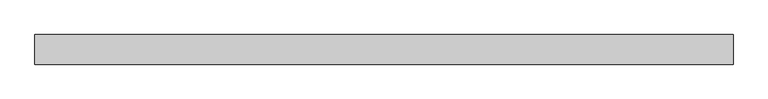
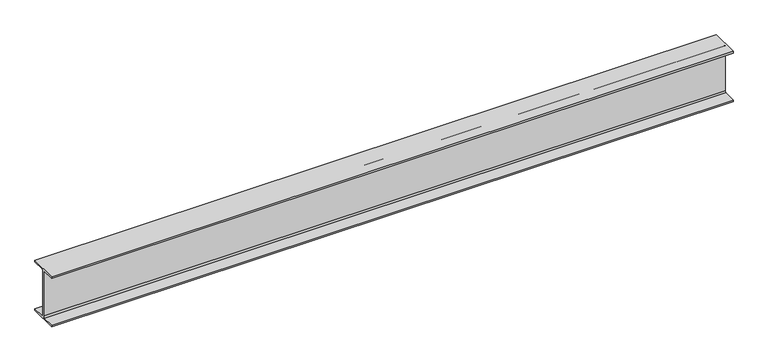
"""IFC4 building model written with IfcOpenShell, lengths in millimetres: beam geometry, Old_Steel Beam_H-KSD3502 : H_SB_ASB_H-250×125x6x9."""

import ifcopenshell
import ifcopenshell.guid

model = None  # the IFC model being written
_history = None  # IfcOwnerHistory: only IFC2X3 demands one
_inside = {}  # id of a spatial element -> (the spatial element, [elements in it])
_under = {}  # id of a project, library or spatial element -> (it, [spatial elements below it])
_declared = {}  # id of a project -> (the project, [libraries it declares])
_typed = {}  # id of a type object -> (the type object, [elements of that type])
_made_of = {}  # id of a material, layer set ... -> (it, [elements and type objects made of it])


def new_model(schema):
    """Start an empty IFC model of exactly this schema.

    Asked for "IFC4X3", IfcOpenShell would pick the latest addendum, in which some entities
    have other attributes; the version numbers below select the first issue.
    IFC2X3 requires an IfcOwnerHistory on every rooted entity: one is made here for all.
    """
    global model, _history
    if schema == "IFC4X3":
        model = ifcopenshell.file(schema_version=(4, 3, 0, 0))
    else:
        model = ifcopenshell.file(schema=schema)
    _inside.clear()
    _under.clear()
    _declared.clear()
    _typed.clear()
    _made_of.clear()
    _history = None
    if model.schema == "IFC2X3":
        org = make("IfcOrganization", Name="unknown")
        user = make(
            "IfcPersonAndOrganization",
            ThePerson=make("IfcPerson", FamilyName="unknown"),
            TheOrganization=org,
        )
        app = make(
            "IfcApplication",
            ApplicationDeveloper=org,
            Version="unknown",
            ApplicationFullName="unknown",
            ApplicationIdentifier="unknown",
        )
        _history = make(
            "IfcOwnerHistory",
            OwningUser=user,
            OwningApplication=app,
            ChangeAction="ADDED",
            CreationDate=0,
        )
    return model


def make(cls, **values):
    """One entity of the class cls with the attributes given. An attribute that is None is left unset."""
    return model.create_entity(
        cls, **{name: value for name, value in values.items() if value is not None}
    )


def rooted(cls, **values):
    """An entity with a GlobalId (a new one), such as an element, a storey or a relation."""
    return make(cls, GlobalId=ifcopenshell.guid.new(), OwnerHistory=_history, **values)


def si_unit(unit_type, name, prefix=None):
    """IfcSIUnit, for example si_unit("LENGTHUNIT", "METRE", prefix="MILLI")."""
    return make("IfcSIUnit", UnitType=unit_type, Prefix=prefix, Name=name)


def assignment(units):
    """IfcUnitAssignment: the units of a project."""
    return None if units is None else make("IfcUnitAssignment", Units=units)


def point(xyz):
    """IfcCartesianPoint."""
    return None if xyz is None else make("IfcCartesianPoint", Coordinates=xyz)


def direction(xyz):
    """IfcDirection."""
    return None if xyz is None else make("IfcDirection", DirectionRatios=xyz)


def frame(location, z_axis=None, x_axis=None):
    """IfcAxis2Placement3D, a coordinate frame: its origin and axes. An axis left out is left unset."""
    return make(
        "IfcAxis2Placement3D",
        Location=point(location),
        Axis=direction(z_axis),
        RefDirection=direction(x_axis),
    )


def frame_2d(location, x_axis=None):
    """IfcAxis2Placement2D, a coordinate frame in the plane: its origin and x axis."""
    return make(
        "IfcAxis2Placement2D", Location=point(location), RefDirection=direction(x_axis)
    )


def origin():
    """The frame at (0, 0, 0) with its axes left unset."""
    return frame((0.0, 0.0, 0.0))


def place(relative_to, where):
    """IfcLocalPlacement: puts the frame where relative to a parent placement (None: the world)."""
    return make(
        "IfcLocalPlacement", PlacementRelTo=relative_to, RelativePlacement=where
    )


def context(
    kind, dimensions, precision=None, world=None, true_north=None, identifier=None
):
    """IfcGeometricRepresentationContext, for example the 3D "Model" context."""
    return make(
        "IfcGeometricRepresentationContext",
        ContextIdentifier=identifier,
        ContextType=kind,
        CoordinateSpaceDimension=dimensions,
        Precision=precision,
        WorldCoordinateSystem=world,
        TrueNorth=true_north,
    )


def project(units=None, contexts=None):
    """IfcProject with its units and contexts."""
    return rooted(
        "IfcProject",
        Name="project",
        RepresentationContexts=contexts,
        UnitsInContext=assignment(units),
    )


def spatial(cls, under=None, at=None, **own):
    """A site, building, storey or space (cls), placed at a placement, below another one or the project."""
    s = rooted(cls, ObjectPlacement=at, **own)
    if under is not None:
        _under.setdefault(under.id(), (under, []))[1].append(s)
    return s


def polyline(points):
    """IfcPolyline through the points."""
    return make("IfcPolyline", Points=[point(p) for p in points])


def circle_curve(where, radius):
    """IfcCircle in the frame where."""
    return make("IfcCircle", Position=where, Radius=radius)


def trimmed(basis, trim1, trim2, sense, master):
    """IfcTrimmedCurve: the piece of a basis curve between two trims."""
    return make(
        "IfcTrimmedCurve",
        BasisCurve=basis,
        Trim1=trim1,
        Trim2=trim2,
        SenseAgreement=sense,
        MasterRepresentation=master,
    )


def segment(curve, same_sense, transition):
    """IfcCompositeCurveSegment."""
    return make(
        "IfcCompositeCurveSegment",
        Transition=transition,
        SameSense=same_sense,
        ParentCurve=curve,
    )


def composite_curve(segments, self_intersect=None):
    """IfcCompositeCurve: segments joined end to end."""
    return make("IfcCompositeCurve", Segments=segments, SelfIntersect=self_intersect)


def outline(outer, holes=None, kind="AREA"):
    """IfcArbitraryClosedProfileDef: a profile drawn as a closed curve; with holes, ...WithVoids."""
    if holes is None:
        return make("IfcArbitraryClosedProfileDef", ProfileType=kind, OuterCurve=outer)
    return make(
        "IfcArbitraryProfileDefWithVoids",
        ProfileType=kind,
        OuterCurve=outer,
        InnerCurves=holes,
    )


def extrude(swept, where, along, depth):
    """IfcExtrudedAreaSolid: the profile swept, set in the frame where, extruded along a direction by depth."""
    return make(
        "IfcExtrudedAreaSolid",
        SweptArea=swept,
        Position=where,
        ExtrudedDirection=direction(along),
        Depth=depth,
    )


def shape(context_of_items, identifier, shape_type, items):
    """IfcShapeRepresentation: the items that make up one representation, for example the "Body"."""
    return make(
        "IfcShapeRepresentation",
        ContextOfItems=context_of_items,
        RepresentationIdentifier=identifier,
        RepresentationType=shape_type,
        Items=items,
    )


def source(mapping_origin, context_of_items, identifier, shape_type, items):
    """IfcRepresentationMap: a shape defined once, which mapped items show again and again."""
    return make(
        "IfcRepresentationMap",
        MappingOrigin=mapping_origin,
        MappedRepresentation=shape(context_of_items, identifier, shape_type, items),
    )


def transform(
    local_origin,
    x_axis=None,
    y_axis=None,
    z_axis=None,
    scale=None,
    scale2=None,
    scale3=None,
    uniform=True,
):
    """IfcCartesianTransformationOperator3D, or its non-uniform kind. x_axis, y_axis, z_axis: its Axis1, 2, 3."""
    if uniform:
        return make(
            "IfcCartesianTransformationOperator3D",
            Axis1=direction(x_axis),
            Axis2=direction(y_axis),
            LocalOrigin=point(local_origin),
            Scale=scale,
            Axis3=direction(z_axis),
        )
    return make(
        "IfcCartesianTransformationOperator3DnonUniform",
        Axis1=direction(x_axis),
        Axis2=direction(y_axis),
        LocalOrigin=point(local_origin),
        Scale=scale,
        Axis3=direction(z_axis),
        Scale2=scale2,
        Scale3=scale3,
    )


def mapped(mapping_source, mapping_target):
    """IfcMappedItem: shows the shape of a source again, moved by a transform."""
    return make(
        "IfcMappedItem", MappingSource=mapping_source, MappingTarget=mapping_target
    )


def made_of(thing, what):
    """Note that an element or type object is made of a material, layer set ...; save() writes the relation."""
    if what is not None:
        _made_of.setdefault(what.id(), (what, []))[1].append(thing)
    return thing


def element(
    cls,
    number,
    at=None,
    inside=None,
    cuts=None,
    type_object=None,
    material=None,
    context=None,
    identifier="Body",
    shape_type=None,
    held_by="IfcProductDefinitionShape",
    body=None,
    shapes=None,
    **own,
):
    """One element of the class cls, such as IfcWall. Its Tag is "e" and its number.

    at: its placement. inside: the storey or other place that contains it. cuts: it is an
    opening in that element (IfcRelVoidsElement). A single representation is given by context,
    identifier, shape_type and body (its items); several are given by shapes. held_by: the class
    of the entity that holds the representations. save() writes the other relations.
    """
    e = rooted(cls, Tag="e%d" % number, ObjectPlacement=at, **own)
    if body is not None:
        shapes = [shape(context, identifier, shape_type, body)]
    if shapes is not None:
        e.Representation = make(held_by, Representations=shapes)
    if inside is not None:
        _inside.setdefault(inside.id(), (inside, []))[1].append(e)
    if cuts is not None:
        rooted(
            "IfcRelVoidsElement", RelatingBuildingElement=cuts, RelatedOpeningElement=e
        )
    if type_object is not None:
        _typed.setdefault(type_object.id(), (type_object, []))[1].append(e)
    return made_of(e, material)


def aggregate(whole, parts):
    """IfcRelAggregates: a whole, such as a stair, and the parts it consists of."""
    return rooted("IfcRelAggregates", RelatingObject=whole, RelatedObjects=parts)


def save(model, path):
    """Write the relations noted so far, then the file.

    IfcRelAggregates (storeys below a building ...), IfcRelContainedInSpatialStructure (elements
    in a storey), IfcRelDefinesByType, IfcRelAssociatesMaterial and IfcRelDeclares: one each for
    every whole, place, type object, material and project.
    """
    for whole, parts in _under.values():
        aggregate(whole, parts)
    for where, things in _inside.values():
        rooted(
            "IfcRelContainedInSpatialStructure",
            RelatedElements=things,
            RelatingStructure=where,
        )
    for kind, things in _typed.values():
        rooted("IfcRelDefinesByType", RelatedObjects=things, RelatingType=kind)
    for what, things in _made_of.values():
        rooted("IfcRelAssociatesMaterial", RelatedObjects=things, RelatingMaterial=what)
    for by, libraries in _declared.values():
        rooted("IfcRelDeclares", RelatingContext=by, RelatedDefinitions=libraries)
    model.write(path)


def beam_36457d38(model_context):
    return source(origin(), model_context, "Body", "SweptSolid", [
        extrude(outline(composite_curve([segment(polyline([(82.5, -141.5), (82.5, -151.7), (-82.5, -151.7), (-82.5, -141.5), (-11.9, -141.5)]), True, "CONTINUOUS"), segment(trimmed(circle_curve(frame_2d((-11.9, -132.6)), 8.9), [point((-11.9, -141.5))], [point((-3.0, -132.6))], True, "CARTESIAN"), True, "CONTINUOUS"), segment(polyline([(-3.0, -132.6), (-3.0, 132.6)]), True, "CONTINUOUS"), segment(trimmed(circle_curve(frame_2d((-11.9, 132.6)), 8.9), [point((-3.0, 132.6))], [point((-11.9, 141.5))], True, "CARTESIAN"), True, "CONTINUOUS"), segment(polyline([(-11.9, 141.5), (-82.5, 141.5), (-82.5, 151.7), (82.5, 151.7), (82.5, 141.5), (11.9, 141.5)]), True, "CONTINUOUS"), segment(trimmed(circle_curve(frame_2d((11.9, 132.6)), 8.9), [point((11.9, 141.5))], [point((3.0, 132.6))], True, "CARTESIAN"), True, "CONTINUOUS"), segment(polyline([(3.0, 132.6), (3.0, -132.6)]), True, "CONTINUOUS"), segment(trimmed(circle_curve(frame_2d((11.9, -132.6)), 8.9), [point((3.0, -132.6))], [point((11.9, -141.5))], True, "CARTESIAN"), True, "CONTINUOUS"), segment(polyline([(11.9, -141.5), (82.5, -141.5)]), True, "CONTINUOUS")], self_intersect=False)), frame((-1904.8, 0.0, 0.0), z_axis=(1.0, 0.0, 0.0), x_axis=(0.0, 1.0, 0.0)), (0.0, 0.0, 1.0), 3892.0999994),
    ])


if __name__ == "__main__":
    model = new_model("IFC4")
    model_context = context("Model", 3, world=origin())
    ifc_project = project(units=[si_unit("LENGTHUNIT", "METRE", prefix="MILLI")], contexts=[model_context])
    site = spatial("IfcSite", under=ifc_project)
    building = spatial("IfcBuilding", under=site)
    placement = place(None, origin())
    beam_shape = beam_36457d38(model_context)
    element("IfcBeam", 1, ObjectType="Old_Steel Beam_H-KSD3502 : H_SB_ASB_H-250×125x6x9", at=placement, inside=building, context=model_context, shape_type="MappedRepresentation", body=[
        mapped(beam_shape, transform((0.0, 0.0, 0.0), x_axis=(1.0, 0.0, 0.0), y_axis=(0.0, 1.0, 0.0), z_axis=(0.0, 0.0, 1.0))),
    ])
    save(model, "model.ifc")

# Revit data of these elements
# Type "Old_Steel Beam_H-KSD3502 : H_SB_ASB_H-250×125x6x9"
#   Width = 12.5 cm
#   Web Thickness = 0.6 cm
#   Web Fillet = 1.2 cm
#   Warping Constant = 42539.8 cm⁶
#   Torsional Moment of Inertia = 7.8102 cm⁴
#   Torsional Modulus = 1.0 cm³
#   Section Area = 37.66 cm²
#   Plastic Modulus weak axis = 73.1 cm³
#   Plastic Modulus strong axis = 366.0 cm³
#   Perimeter = 0.97 m²/m
#   Nominal Weight = 29.60 kgf/m
#   Moment of Inertia weak axis = 294.00 cm⁴
#   Moment of Inertia strong axis = 4050.00 cm⁴
#   Height = 25.0 cm
#   Flange Thickness = 0.9 cm
#   Elastic Modulus weak axis = 47.0 cm³
#   Elastic Modulus strong axis = 324.0 cm³
#   Centroid Vertical = 12.5 cm
#   Centroid Horizontal = 6.25 cm
#   Length [instance default] = 1.5240 m
#   Structural Material [instance default] = Steel, 45-345
#   Assembly Code = ""
# Element 1 (IfcBeam, "Old_Steel Beam_H-KSD3502 : H_SB_ASB_H-250×125x6x9")
#   Structural Material = none
# Materials
#   "Steel, 45-345": class "Metal", colour RGB 189 187 185, transparency 0, Description = "Steel 345 MPa", Cost = 0
